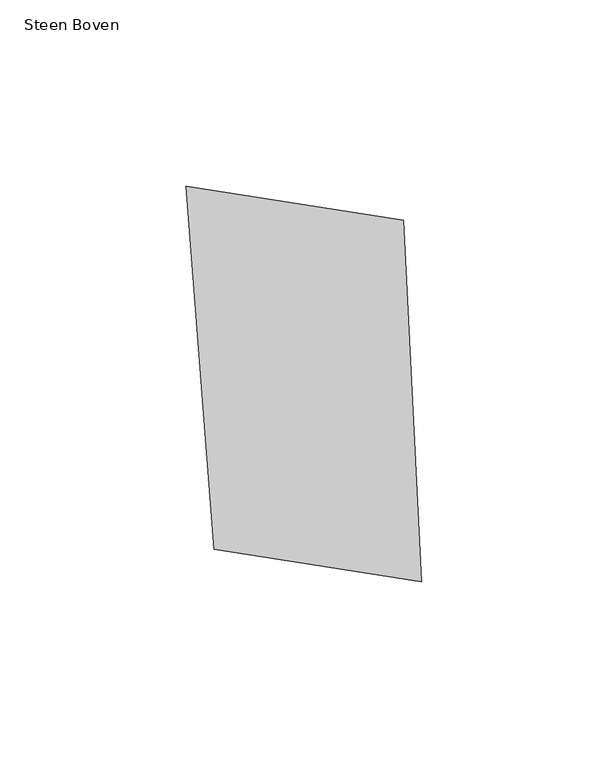
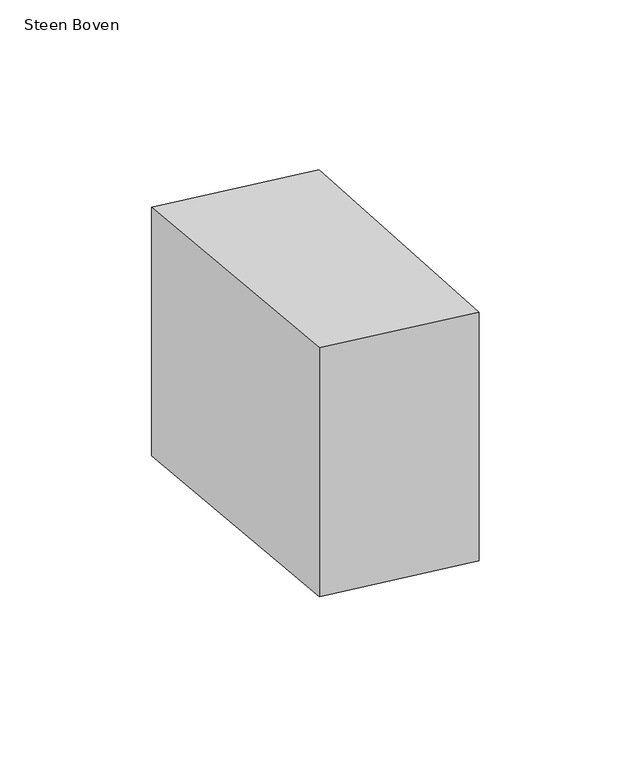
"""IFC4 building model written with IfcOpenShell, lengths in millimetres: proxy geometry, 00_GMA_steen_versie_4 : Steen Boven."""

from ifc_helpers import new_model, si_unit, origin, origin_with_axes, place, context, project, spatial, polyline, outline, extrude, source, transform, mapped, element, save


def steen_boven_5877faa3(model_context):
    return source(origin(), model_context, "Body", "SweptSolid", [
        extrude(outline(polyline([(98.0487886, 120.3567909), (102.9241546, 23.3592647), (47.2500623, 31.9653486), (39.7792327, 129.3895689), (98.0487886, 120.3567909)])), origin_with_axes(), (0.0, 0.0, 1.0), 100.0),
    ])


if __name__ == "__main__":
    model = new_model("IFC4")
    model_context = context("Model", 3, world=origin())
    ifc_project = project(units=[si_unit("LENGTHUNIT", "METRE", prefix="MILLI")], contexts=[model_context])
    site = spatial("IfcSite", under=ifc_project)
    building = spatial("IfcBuilding", under=site)
    placement = place(None, origin())
    steen_boven_shape = steen_boven_5877faa3(model_context)
    element("IfcBuildingElementProxy", 1, Name="00_GMA_steen_versie_4 : Steen Boven", ObjectType="00_GMA_steen_versie_4 : Steen Boven", at=placement, inside=building, context=model_context, shape_type="MappedRepresentation", body=[
        mapped(steen_boven_shape, transform((0.0, 0.0, 0.0), x_axis=(1.0, 0.0, 0.0), y_axis=(0.0, 1.0, 0.0), z_axis=(0.0, 0.0, 1.0))),
    ])
    save(model, "model.ifc")

# Revit data of these elements
# Type "00_GMA_steen_versie_4 : Steen Boven"
#   StootVoegHalfBoven [instance default] = 5 mm
#   StootVoegHalf [instance default] = 5 mm
#   StootVoegBreedteOnder = 10 mm
#   StootVoegBreedteBoven = 10 mm
#   Steendikte = 100 mm
#   LintVoegOnderHalf = 5 mm
#   LintVoegOnder = 10 mm
#   LintVoegBovenHalf = 0 mm
#   LintVoegBoven = 0 mm
#   materiaal = none
#   MateriaalVoeg = none
#   Default Elevation = 0
